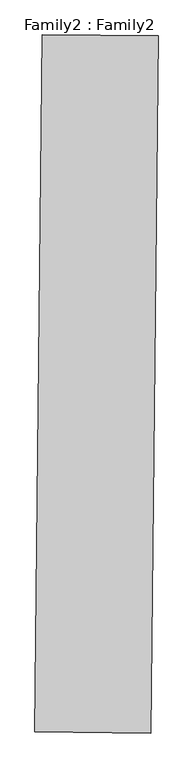
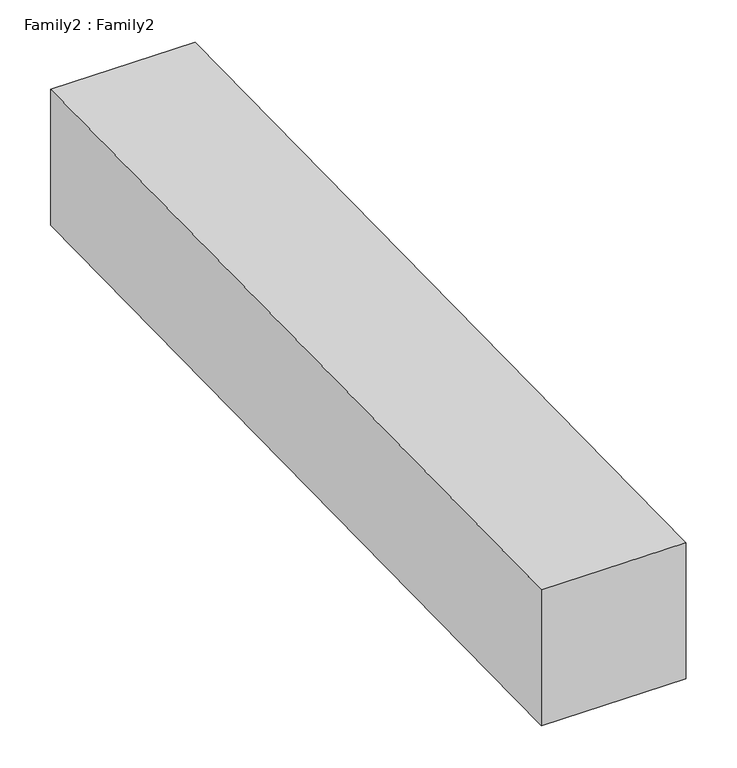
"""IFC4 building model written with IfcOpenShell, lengths in millimetres: proxy geometry, Family2 : Family2."""

from ifc_helpers import new_model, si_unit, origin, place, context, project, spatial, faceted_brep, source, transform, mapped, element, save


def family2_family2_e0ce6eab(model_context):
    return source(origin(), model_context, "Body", "Brep", [
        faceted_brep([(-3949.895153, -6676.7082402, 1.0945136), (-3949.895153, -6676.7082402, 201.0945136), (-3936.9476415, -5470.8918824, 202.060409), (-3936.9476415, -5470.8918824, 2.060409), (-3749.903963, -6678.5854529, 201.0945136), (-3736.9564515, -5472.769095, 202.060409), (-3749.903963, -6678.5854529, 1.0945136), (-3736.9564515, -5472.769095, 2.060409)], [[[0, 1, 2, 3]], [[1, 4, 5, 2]], [[4, 6, 7, 5]], [[6, 0, 3, 7]], [[3, 2, 5, 7]], [[0, 6, 4, 1]]]),
    ])


if __name__ == "__main__":
    model = new_model("IFC4")
    model_context = context("Model", 3, world=origin())
    ifc_project = project(units=[si_unit("LENGTHUNIT", "METRE", prefix="MILLI")], contexts=[model_context])
    site = spatial("IfcSite", under=ifc_project)
    building = spatial("IfcBuilding", under=site)
    placement = place(None, origin())
    family2_family2_shape = family2_family2_e0ce6eab(model_context)
    element("IfcBuildingElementProxy", 1, Name="Family2 : Family2", ObjectType="Family2 : Family2", at=placement, inside=building, context=model_context, shape_type="MappedRepresentation", body=[
        mapped(family2_family2_shape, transform((0.0, 0.0, 0.0), x_axis=(1.0, 0.0, 0.0), y_axis=(0.0, 1.0, 0.0), z_axis=(0.0, 0.0, 1.0))),
    ])
    save(model, "model.ifc")

# Revit data of these elements
# Type "Family2 : Family2"
#   Default Elevation = 0
